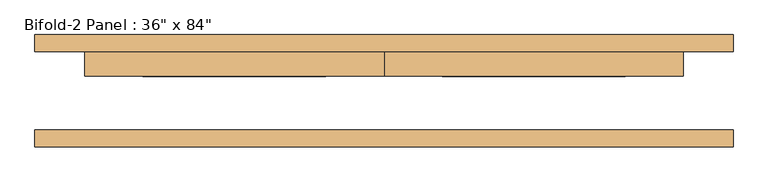
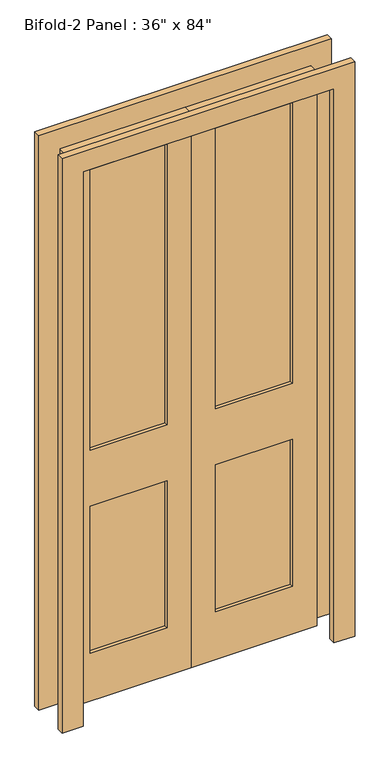
"""IFC4 building model written with IfcOpenShell, lengths in millimetres: door geometry."""

from ifc_helpers import new_model, si_unit, frame, origin, place, context, project, spatial, polyline, outline, extrude, source, transform, mapped, element, save


def door_80e19791(model_context):
    return source(origin(), model_context, "Body", "SweptSolid", [
        extrude(outline(polyline([(2133.6, 0.0), (2133.6, -457.2), (0.0, -457.2), (0.0, 0.0), (2133.6, 0.0)]), holes=[polyline([(2044.7, -88.9), (965.11872, -88.9), (965.11872, -368.3), (2044.7, -368.3), (2044.7, -88.9)]), polyline([(749.3, -88.9), (184.15, -88.9), (184.15, -368.3), (749.3, -368.3), (749.3, -88.9)])]), frame((0.0, 22.225, 0.0), z_axis=(0.0, 1.0, 0.0), x_axis=(0.0, 0.0, 1.0)), (0.0, 0.0, 1.0), 38.1),
        extrude(outline(polyline([(-88.9, 34.925), (-368.3, 34.925), (-368.3, 47.625), (-88.9, 47.625), (-88.9, 34.925)])), frame((0.0, 0.0, 965.11872), z_axis=(0.0, 0.0, 1.0), x_axis=(1.0, 0.0, 0.0)), (0.0, 0.0, 1.0), 1079.58128),
        extrude(outline(polyline([(-88.9, 34.925), (-368.3, 34.925), (-368.3, 47.625), (-88.9, 47.625), (-88.9, 34.925)])), frame((0.0, 0.0, 184.15), z_axis=(0.0, 0.0, 1.0), x_axis=(1.0, 0.0, 0.0)), (0.0, 0.0, 1.0), 565.15),
        extrude(outline(polyline([(368.3, 34.925), (88.9, 34.925), (88.9, 47.625), (368.3, 47.625), (368.3, 34.925)])), frame((0.0, 0.0, 965.11872), z_axis=(0.0, 0.0, 1.0), x_axis=(1.0, 0.0, 0.0)), (0.0, 0.0, 1.0), 1079.58128),
        extrude(outline(polyline([(368.3, 34.925), (88.9, 34.925), (88.9, 47.625), (368.3, 47.625), (368.3, 34.925)])), frame((0.0, 0.0, 184.15), z_axis=(0.0, 0.0, 1.0), x_axis=(1.0, 0.0, 0.0)), (0.0, 0.0, 1.0), 565.15),
        extrude(outline(polyline([(2209.8, -533.4), (0.0, -533.4), (0.0, -457.2), (2133.6, -457.2), (2133.6, 457.2), (0.0, 457.2), (0.0, 533.4), (2209.8, 533.4), (2209.8, -533.4)])), frame((0.0, 60.325, 0.0), z_axis=(0.0, 1.0, 0.0), x_axis=(0.0, 0.0, 1.0)), (0.0, 0.0, 1.0), 25.4),
        extrude(outline(polyline([(2209.8, 533.4), (2209.8, -533.4), (0.0, -533.4), (0.0, -457.2), (2133.6, -457.2), (2133.6, 457.2), (0.0, 457.2), (0.0, 533.4), (2209.8, 533.4)])), frame((0.0, -85.725, 0.0), z_axis=(0.0, 1.0, 0.0), x_axis=(0.0, 0.0, 1.0)), (0.0, 0.0, 1.0), 25.4),
        extrude(outline(polyline([(2133.6, 457.2), (2133.6, 0.0), (0.0, 0.0), (0.0, 457.2), (2133.6, 457.2)]), holes=[polyline([(2044.7, 88.9), (2044.7, 368.3), (965.11872, 368.3), (965.11872, 88.9), (2044.7, 88.9)]), polyline([(749.3, 88.9), (749.3, 368.3), (184.15, 368.3), (184.15, 88.9), (749.3, 88.9)])]), frame((0.0, 22.225, 0.0), z_axis=(0.0, 1.0, 0.0), x_axis=(0.0, 0.0, 1.0)), (0.0, 0.0, 1.0), 38.1),
    ])


if __name__ == "__main__":
    model = new_model("IFC4")
    model_context = context("Model", 3, world=origin())
    ifc_project = project(units=[si_unit("LENGTHUNIT", "METRE", prefix="MILLI")], contexts=[model_context])
    site = spatial("IfcSite", under=ifc_project)
    building = spatial("IfcBuilding", under=site)
    placement = place(None, origin())
    door_shape = door_80e19791(model_context)
    element("IfcDoor", 1, ObjectType="Bifold-2 Panel : 36\" x 84\"", at=placement, inside=building, context=model_context, shape_type="MappedRepresentation", body=[
        mapped(door_shape, transform((0.0, 0.0, 0.0), x_axis=(1.0, 0.0, 0.0), y_axis=(0.0, 1.0, 0.0), z_axis=(0.0, 0.0, 1.0))),
    ])
    save(model, "model.ifc")

# Revit data of these elements
# Type "Bifold-2 Panel : 36\" x 84\""
#   Type Mark = "8"
#   Construction Type Id = "MDOOR"
#   Assembly Code = "C1020"
#   Analytic Construction = "Metal"
#   Thickness = 0' - 1 1/2"
#   Thermal Resistance (R) = 1.5338 (h·ft²·°F)/BTU
#   Heat Transfer Coefficient (U) = 0.651978 BTU/(h·ft²·°F)
#   Height = 7' - 0"
#   Trim Projection Ext = 0' - 1"
#   Trim Projection Int = 0' - 1"
#   Trim Width = 0' - 3"
#   Width = 3' - 0"
#   Define Thermal Properties by = 1
#   Door Material = Door - Panel
#   Frame Material = Door - Frame
#   Visual Light Transmittance = 0
#   Solar Heat Gain Coefficient = 0
#   Function = (empty or 0)
#   Wall Closure = (empty or 0)
# Element 1 (IfcDoor, "Bifold-2 Panel : 36\" x 84\"")
#   Materials on its faces: "Door - Panel", "Door - Frame"
# Materials
#   "Door - Panel": class "Wood", colour RGB 210 159 95, transparency 0, Cost = 0
#   "Door - Frame": class "Miscellaneous", colour RGB 118 70 51, transparency 0, Cost = 0
